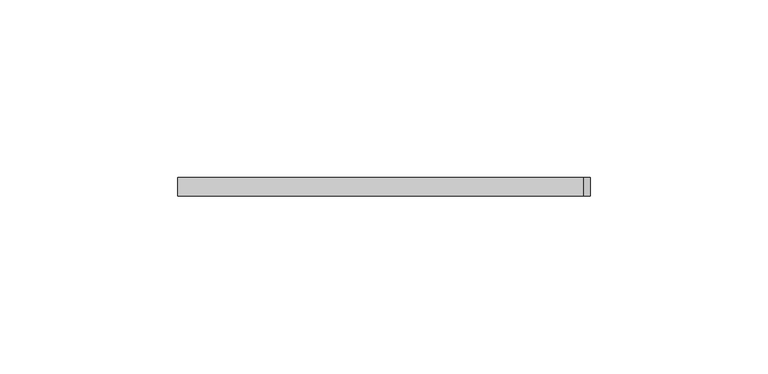
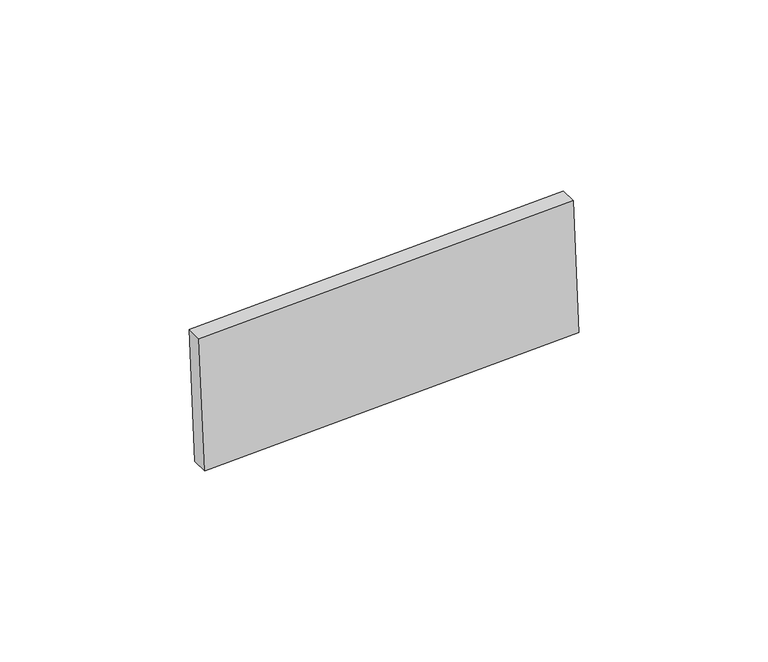
"""IFC4 building model written with IfcOpenShell, lengths in millimetres: proxy geometry, Inner panel:Inner panel:1:Inner panel:1 : Inner panel:Inner panel:300324:2:Inner panel:1:Inner panel:1 : Inner panel:Inner panel:300324:2 : Inner panel:Inner panel:1:Inner panel:1 : Inner panel:Inner panel:300324:300043:166 : Inner panel:Inner panel:1:Inner panel:1 : Inner panel:Inner panel:300324:2:Inner panel:1:Inner panel:1 : Inner panel:Inner panel:300324:2 : Inner panel:Inner panel:1:Inner panel:1 : Inner panel:Inner panel:300324:300043:308120."""

from ifc_helpers import new_model, si_unit, frame, origin, place, context, project, spatial, polyline, outline, extrude, source, transform, mapped, element, save


def generic_models_52687253(model_context):
    return source(origin(), model_context, "Body", "SweptSolid", [
        extrude(outline(polyline([(0.0, -114.3), (0.0, 0.0), (5.213809, 0.0), (5.213809, -114.3), (0.0, -114.3)])), frame((560425.2415304, -564994.107991, 3954.8593665), z_axis=(-0.04163054471216399, 0.0, 0.9991330730923527), x_axis=(0.0, -1.0, 0.0)), (0.0, 0.0, 1.0), 43.2233908),
    ])


if __name__ == "__main__":
    model = new_model("IFC4")
    model_context = context("Model", 3, world=origin())
    ifc_project = project(units=[si_unit("LENGTHUNIT", "METRE", prefix="MILLI")], contexts=[model_context])
    site = spatial("IfcSite", under=ifc_project)
    building = spatial("IfcBuilding", under=site)
    placement = place(None, origin())
    generic_models_shape = generic_models_52687253(model_context)
    element("IfcBuildingElementProxy", 1, Name="Inner panel:Inner panel:1:Inner panel:1 : Inner panel:Inner panel:300324:2:Inner panel:1:Inner panel:1 : Inner panel:Inner panel:300324:2 : Inner panel:Inner panel:1:Inner panel:1 : Inner panel:Inner panel:300324:300043:166 : Inner panel:Inner panel:1:Inner panel:1 : Inner panel:Inner panel:300324:2:Inner panel:1:Inner panel:1 : Inner panel:Inner panel:300324:2 : Inner panel:Inner panel:1:Inner panel:1 : Inner panel:Inner panel:300324:300043:308120", ObjectType="Inner panel:Inner panel:1:Inner panel:1 : Inner panel:Inner panel:300324:2:Inner panel:1:Inner panel:1 : Inner panel:Inner panel:300324:2 : Inner panel:Inner panel:1:Inner panel:1 : Inner panel:Inner panel:300324:300043:166 : Inner panel:Inner panel:1:Inner panel:1 : Inner panel:Inner panel:300324:2:Inner panel:1:Inner panel:1 : Inner panel:Inner panel:300324:2 : Inner panel:Inner panel:1:Inner panel:1 : Inner panel:Inner panel:300324:300043:308120", at=placement, inside=building, context=model_context, shape_type="MappedRepresentation", body=[
        mapped(generic_models_shape, transform((0.0, 0.0, 0.0), x_axis=(1.0, 0.0, 0.0), y_axis=(0.0, 1.0, 0.0), z_axis=(0.0, 0.0, 1.0))),
    ])
    save(model, "model.ifc")

# Revit data of these elements
# Type "Inner panel:Inner panel:1:Inner panel:1 : Inner panel:Inner panel:300324:2:Inner panel:1:Inner panel:1 : Inner panel:Inner panel:300324:2 : Inner panel:Inner panel:1:Inner panel:1 : Inner panel:Inner panel:300324:300043:166 : Inner panel:Inner panel:1:Inner panel:1 : Inner panel:Inner panel:300324:2:Inner panel:1:Inner panel:1 : Inner panel:Inner panel:300324:2 : Inner panel:Inner panel:1:Inner panel:1 : Inner panel:Inner panel:300324:300043:308120"
#   NameOverride = "Inner panel:Inner panel:1:Inner panel:1 : Inner panel:Inner panel:300324:2:Inner panel:1:Inner panel:1 : Inner panel:Inner panel:300324:2 : Inner panel:Inner panel:1:Inner panel:1 : Inner panel:Inner panel:300324:300043:308120"
#   ObjectTypeOverride = "Inner panel:1:Inner panel:1 : Inner panel:Inner panel:300324:2 : Inner panel:Inner panel:1:Inner panel:1 : Inner panel:Inner panel:300324:300043"
#   Reference = "Inner panel"
#   Tag = "308120"
# Element 1 (IfcBuildingElementProxy, "Inner panel:Inner panel:1:Inner panel:1 : Inner panel:Inner panel:300324:2:Inner panel:1:Inner panel:1 : Inner panel:Inner panel:300324:2 : Inner panel:Inner panel:1:Inner panel:1 : Inner panel:Inner panel:300324:300043:166 : Inner panel:Inner panel:1:Inner panel:1 : Inner panel:Inner panel:300324:2:Inner panel:1:Inner panel:1 : Inner panel:Inner panel:300324:2 : Inner panel:Inner panel:1:Inner panel:1 : Inner panel:Inner panel:300324:300043:308120")
#   Materials on its faces: "SLIDING CLIP"
# Materials
#   "SLIDING CLIP": class "Generic", colour RGB 120 120 120, transparency 0, Cost = 0
